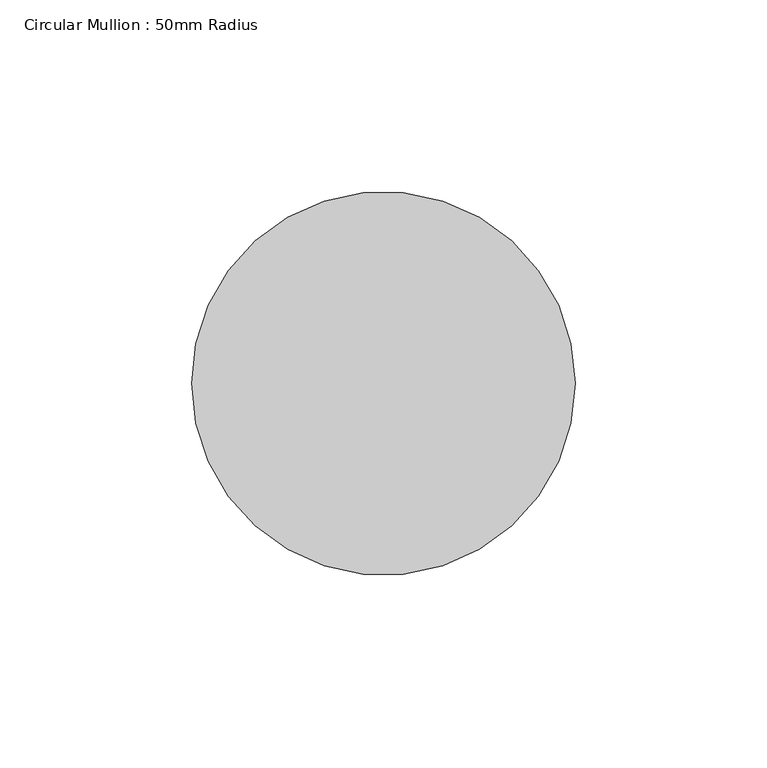
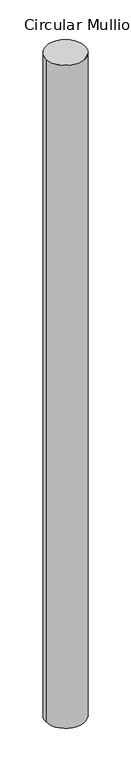
"""IFC4 building model written with IfcOpenShell, lengths in millimetres: member geometry, Circular Mullion : 50mm Radius."""

from ifc_helpers import new_model, si_unit, point, frame, origin, origin_2d, place, context, project, spatial, circle_curve, trimmed, segment, composite_curve, outline, extrude, source, transform, mapped, element, save


def circular_mullion_50mm_radius_08229a83(model_context):
    return source(origin(), model_context, "Body", "SweptSolid", [
        extrude(outline(composite_curve([segment(trimmed(circle_curve(origin_2d(), 50.0), [point((50.0, 0.0))], [point((-50.0, 0.0))], False, "CARTESIAN"), True, "CONTINUOUS"), segment(trimmed(circle_curve(origin_2d(), 50.0), [point((-50.0, 0.0))], [point((50.0, 0.0))], False, "CARTESIAN"), True, "CONTINUOUS")], self_intersect=False)), frame((0.0, 0.0, -1795.1670143), z_axis=(0.0, 0.0, 1.0), x_axis=(1.0, 0.0, 0.0)), (0.0, 0.0, 1.0), 1795.1670143),
    ])


if __name__ == "__main__":
    model = new_model("IFC4")
    model_context = context("Model", 3, world=origin())
    ifc_project = project(units=[si_unit("LENGTHUNIT", "METRE", prefix="MILLI")], contexts=[model_context])
    site = spatial("IfcSite", under=ifc_project)
    building = spatial("IfcBuilding", under=site)
    placement = place(None, origin())
    circular_mullion_50mm_radius_shape = circular_mullion_50mm_radius_08229a83(model_context)
    element("IfcMember", 1, ObjectType="Circular Mullion : 50mm Radius", at=placement, inside=building, context=model_context, shape_type="MappedRepresentation", body=[
        mapped(circular_mullion_50mm_radius_shape, transform((0.0, 0.0, 0.0), x_axis=(1.0, 0.0, 0.0), y_axis=(0.0, 1.0, 0.0), z_axis=(0.0, 0.0, 1.0))),
    ])
    save(model, "model.ifc")

# Revit data of these elements
# Type "Circular Mullion : 50mm Radius"
#   built-in parameter 1007350 = 0.164042 (stored number, unit not read)
# Element 1 (IfcMember, "Circular Mullion : 50mm Radius")
#   Materials on its faces: "Aluminium"
# Materials
#   "Aluminium": class "Metal", colour RGB 247 247 247, transparency 0, Description = "Aluminium 6061", Cost = 0
